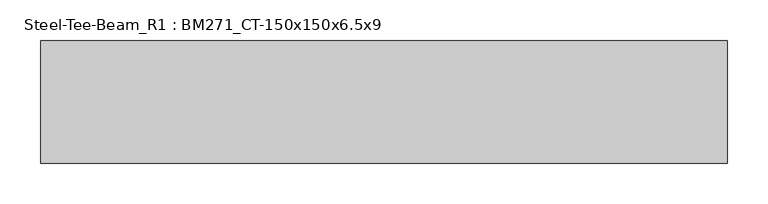
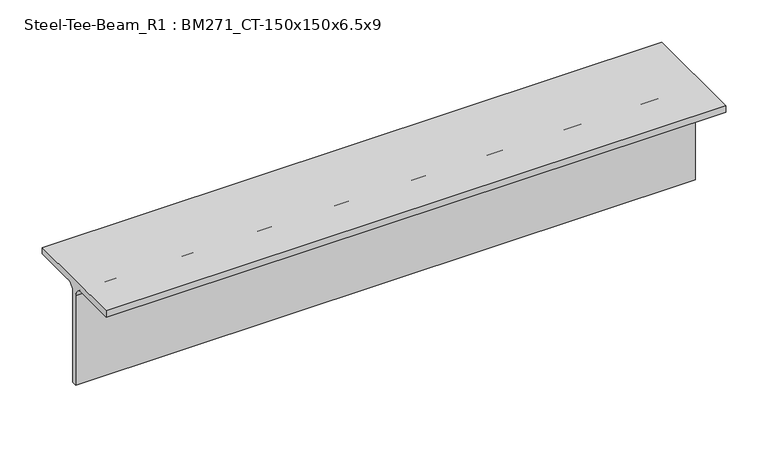
"""IFC4 building model written with IfcOpenShell, lengths in millimetres: member geometry, Steel-Tee-Beam_R1 : BM271_CT-150x150x6.5x9."""

from ifc_helpers import new_model, si_unit, point, frame, frame_2d, origin, place, context, project, spatial, polyline, circle_curve, trimmed, segment, composite_curve, outline, extrude, source, transform, mapped, element, save


def steel_tee_beam_r1_bm271_ct_150x150x6_5x9_6f36bbda(model_context):
    return source(origin(), model_context, "Body", "SweptSolid", [
        extrude(outline(composite_curve([segment(polyline([(75.0, 75.0), (75.0, 66.0), (16.25, 66.0)]), True, "CONTINUOUS"), segment(trimmed(circle_curve(frame_2d((16.25, 53.0)), 13.0), [point((16.25, 66.0))], [point((3.25, 53.0))], True, "CARTESIAN"), True, "CONTINUOUS"), segment(polyline([(3.25, 53.0), (3.25, -75.0), (-3.25, -75.0), (-3.25, 53.0)]), True, "CONTINUOUS"), segment(trimmed(circle_curve(frame_2d((-16.25, 53.0)), 13.0), [point((-3.25, 53.0))], [point((-16.25, 66.0))], True, "CARTESIAN"), True, "CONTINUOUS"), segment(polyline([(-16.25, 66.0), (-75.0, 66.0), (-75.0, 75.0), (75.0, 75.0)]), True, "CONTINUOUS")], self_intersect=False)), frame((-341.5608007, 0.0, 0.0), z_axis=(1.0, 0.0, 0.0), x_axis=(0.0, 1.0, 0.0)), (0.0, 0.0, 1.0), 841.5608007),
    ])


if __name__ == "__main__":
    model = new_model("IFC4")
    model_context = context("Model", 3, world=origin())
    ifc_project = project(units=[si_unit("LENGTHUNIT", "METRE", prefix="MILLI")], contexts=[model_context])
    site = spatial("IfcSite", under=ifc_project)
    building = spatial("IfcBuilding", under=site)
    placement = place(None, origin())
    steel_tee_beam_r1_bm271_ct_150x150x6_5x9_shape = steel_tee_beam_r1_bm271_ct_150x150x6_5x9_6f36bbda(model_context)
    element("IfcMember", 1, ObjectType="Steel-Tee-Beam_R1 : BM271_CT-150x150x6.5x9", at=placement, inside=building, context=model_context, shape_type="MappedRepresentation", body=[
        mapped(steel_tee_beam_r1_bm271_ct_150x150x6_5x9_shape, transform((0.0, 0.0, 0.0), x_axis=(1.0, 0.0, 0.0), y_axis=(0.0, 1.0, 0.0), z_axis=(0.0, 0.0, 1.0))),
    ])
    save(model, "model.ifc")

# Revit data of these elements
# Type "Steel-Tee-Beam_R1 : BM271_CT-150x150x6.5x9"
#   Keynote = "CT-150x150x6.5x9"
#   Surface Area = 0.588841 m²/m
#   Section Area = 23.3904 cm²
#   Mass per Unit Length = 18.3614 kg/m
#   Length [instance default] = 1.5240 m
#   bf = 0.1500 m
#   d = 0.1500 m
#   k = 0.0220 m
#   r = 0.0130 m
#   tf = 0.0090 m
#   tw = 0.0065 m
#   hec_material4 [instance default] = none
#   hec_material3 [instance default] = none
#   hec_material2 [instance default] = none
#   hec_material1 [instance default] = none
#   Structural Material [instance default] = Steel, 45-345
#   Assembly Code = ""
# Element 1 (IfcMember, "Steel-Tee-Beam_R1 : BM271_CT-150x150x6.5x9")
#   Structural Material = none
# Materials
#   "Steel, 45-345": class "Metal", colour RGB 189 187 185, transparency 0, Description = "Steel 345 MPa", Cost = 0
